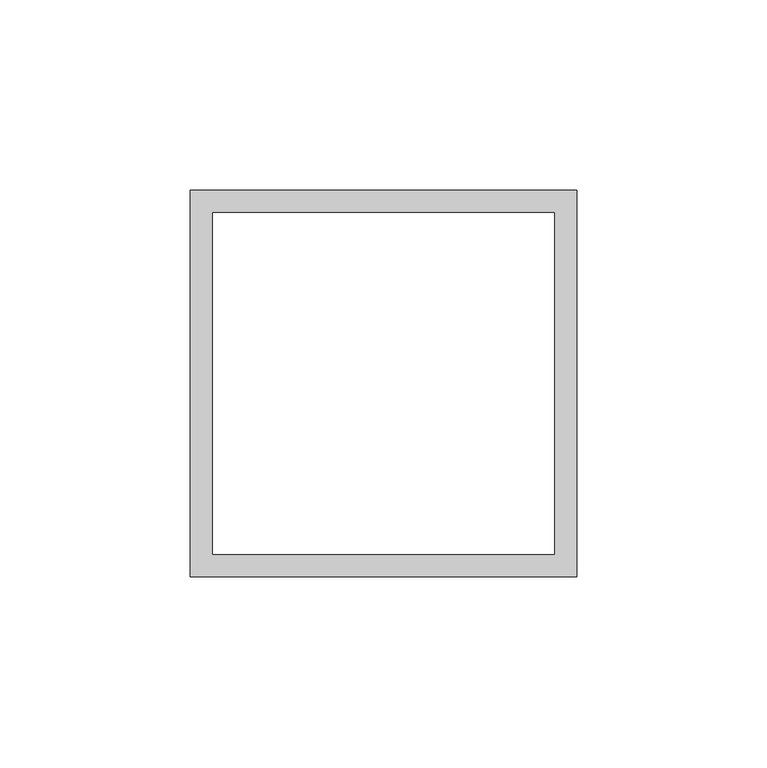
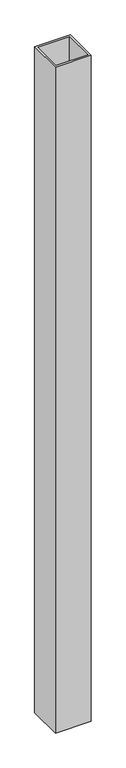
"""IFC4 building model written with IfcOpenShell, lengths in millimetres: proxy geometry, Generic Models 7:Generic Models 1:3:Generic Models 1:3 : Generic Models 7:Generic Models 1:305549:3:Generic Models 1:3:Generic Models 1:3 : Generic Models 7:Generic Models 1:305549:3 : Generic Models 7:Generic Models 1:3:Generic Models 1:3 : Generic Models 7:Generic Models 1:305549:301244:17 : Generic Models 7:Generic Models 1:3:Generic Models 1:3 : Generic Models 7:Generic Models 1:305549:3:Generic Models 1:3:Generic Models 1:3 : Generic Models 7:Generic Models 1:305549:3 : Generic Models 7:Generic Models 1:3:Generic Models 1:3 : Generic Models 7:Generic Models 1:305549:301244:308848."""

from ifc_helpers import new_model, si_unit, frame, origin, place, context, project, spatial, polyline, outline, extrude, source, transform, mapped, element, save


def generic_models_e3ee71aa(model_context):
    return source(origin(), model_context, "Body", "SweptSolid", [
        extrude(outline(polyline([(560619.6617239, -578797.4842061), (560619.6617239, -578899.0842061), (560518.0617239, -578899.0842061), (560518.0617239, -578797.4842061), (560619.6617239, -578797.4842061)]), holes=[polyline([(560613.7435239, -578893.1660061), (560613.7435239, -578803.4024061), (560523.9799239, -578803.4024061), (560523.9799239, -578893.1660061), (560613.7435239, -578893.1660061)])]), frame((0.0, 0.0, 4133.81326), z_axis=(0.0, 0.0, 1.0), x_axis=(1.0, 0.0, 0.0)), (0.0, 0.0, 1.0), 2000.28674),
    ])


if __name__ == "__main__":
    model = new_model("IFC4")
    model_context = context("Model", 3, world=origin())
    ifc_project = project(units=[si_unit("LENGTHUNIT", "METRE", prefix="MILLI")], contexts=[model_context])
    site = spatial("IfcSite", under=ifc_project)
    building = spatial("IfcBuilding", under=site)
    placement = place(None, origin())
    generic_models_shape = generic_models_e3ee71aa(model_context)
    element("IfcBuildingElementProxy", 1, Name="Generic Models 7:Generic Models 1:3:Generic Models 1:3 : Generic Models 7:Generic Models 1:305549:3:Generic Models 1:3:Generic Models 1:3 : Generic Models 7:Generic Models 1:305549:3 : Generic Models 7:Generic Models 1:3:Generic Models 1:3 : Generic Models 7:Generic Models 1:305549:301244:17 : Generic Models 7:Generic Models 1:3:Generic Models 1:3 : Generic Models 7:Generic Models 1:305549:3:Generic Models 1:3:Generic Models 1:3 : Generic Models 7:Generic Models 1:305549:3 : Generic Models 7:Generic Models 1:3:Generic Models 1:3 : Generic Models 7:Generic Models 1:305549:301244:308848", ObjectType="Generic Models 7:Generic Models 1:3:Generic Models 1:3 : Generic Models 7:Generic Models 1:305549:3:Generic Models 1:3:Generic Models 1:3 : Generic Models 7:Generic Models 1:305549:3 : Generic Models 7:Generic Models 1:3:Generic Models 1:3 : Generic Models 7:Generic Models 1:305549:301244:17 : Generic Models 7:Generic Models 1:3:Generic Models 1:3 : Generic Models 7:Generic Models 1:305549:3:Generic Models 1:3:Generic Models 1:3 : Generic Models 7:Generic Models 1:305549:3 : Generic Models 7:Generic Models 1:3:Generic Models 1:3 : Generic Models 7:Generic Models 1:305549:301244:308848", at=placement, inside=building, context=model_context, shape_type="MappedRepresentation", body=[
        mapped(generic_models_shape, transform((0.0, 0.0, 0.0), x_axis=(1.0, 0.0, 0.0), y_axis=(0.0, 1.0, 0.0), z_axis=(0.0, 0.0, 1.0))),
    ])
    save(model, "model.ifc")

# Revit data of these elements
# Type "Generic Models 7:Generic Models 1:3:Generic Models 1:3 : Generic Models 7:Generic Models 1:305549:3:Generic Models 1:3:Generic Models 1:3 : Generic Models 7:Generic Models 1:305549:3 : Generic Models 7:Generic Models 1:3:Generic Models 1:3 : Generic Models 7:Generic Models 1:305549:301244:17 : Generic Models 7:Generic Models 1:3:Generic Models 1:3 : Generic Models 7:Generic Models 1:305549:3:Generic Models 1:3:Generic Models 1:3 : Generic Models 7:Generic Models 1:305549:3 : Generic Models 7:Generic Models 1:3:Generic Models 1:3 : Generic Models 7:Generic Models 1:305549:301244:308848"
#   NameOverride = "Generic Models 7:Generic Models 1:3:Generic Models 1:3 : Generic Models 7:Generic Models 1:305549:3:Generic Models 1:3:Generic Models 1:3 : Generic Models 7:Generic Models 1:305549:3 : Generic Models 7:Generic Models 1:3:Generic Models 1:3 : Generic Models 7:Generic Models 1:305549:301244:308848"
#   ObjectTypeOverride = "Generic Models 1:3:Generic Models 1:3 : Generic Models 7:Generic Models 1:305549:3 : Generic Models 7:Generic Models 1:3:Generic Models 1:3 : Generic Models 7:Generic Models 1:305549:301244"
#   Reference = "Generic Models 1"
#   Tag = "308848"
# Element 1 (IfcBuildingElementProxy, "Generic Models 7:Generic Models 1:3:Generic Models 1:3 : Generic Models 7:Generic Models 1:305549:3:Generic Models 1:3:Generic Models 1:3 : Generic Models 7:Generic Models 1:305549:3 : Generic Models 7:Generic Models 1:3:Generic Models 1:3 : Generic Models 7:Generic Models 1:305549:301244:17 : Generic Models 7:Generic Models 1:3:Generic Models 1:3 : Generic Models 7:Generic Models 1:305549:3:Generic Models 1:3:Generic Models 1:3 : Generic Models 7:Generic Models 1:305549:3 : Generic Models 7:Generic Models 1:3:Generic Models 1:3 : Generic Models 7:Generic Models 1:305549:301244:308848")
#   Materials on its faces: "STRUCTURAL STEEL - SEE STRUCT. DWGS"
# Materials
#   "STRUCTURAL STEEL - SEE STRUCT. DWGS": class "Metal", colour RGB 189 187 185, transparency 0, Description = "Structural steel 50ksi", Cost = 0
